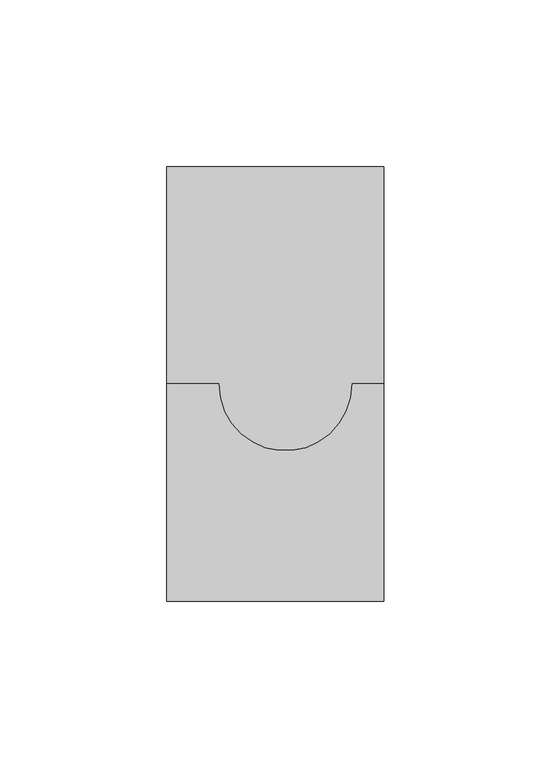
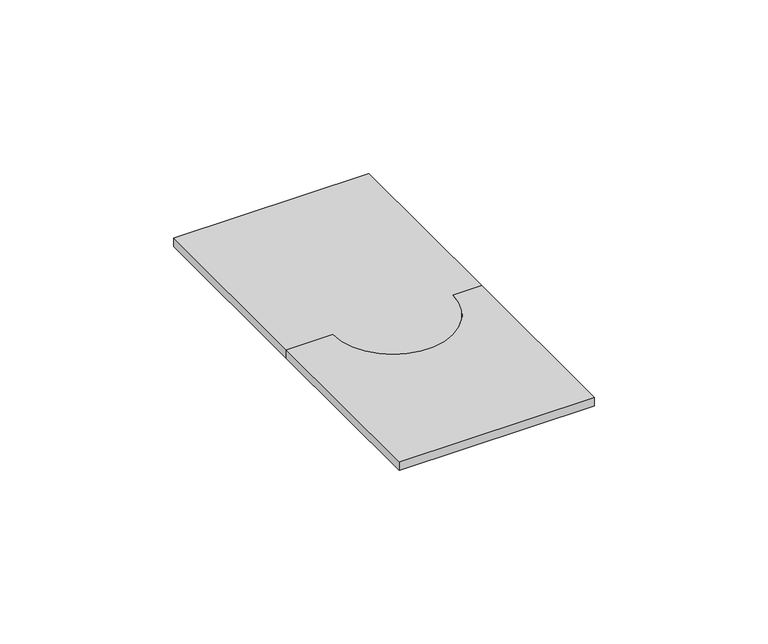
"""IFC4 building model written with IfcOpenShell, lengths in millimetres: proxy geometry, TSP Bonding & Earthing : TSP Bonding & Earthing."""

from ifc_helpers import new_model, si_unit, point, frame_2d, origin, origin_with_axes, place, context, project, spatial, polyline, circle_curve, trimmed, segment, composite_curve, outline, extrude, source, transform, mapped, element, save


def electrical_fixtures_1672ed60(model_context):
    return source(origin(), model_context, "Body", "SweptSolid", [
        extrude(outline(composite_curve([segment(polyline([(-9.5215648, 0.0), (0.0, 0.0), (0.0, -65.0), (-65.0, -65.0), (-65.0, 0.0), (-49.5215648, 0.0)]), True, "CONTINUOUS"), segment(trimmed(circle_curve(frame_2d((-29.5215648, 0.0)), 20.0), [point((-49.5215648, 0.0))], [point((-9.5215648, 0.0))], True, "CARTESIAN"), True, "CONTINUOUS")], self_intersect=False)), origin_with_axes(), (0.0, 0.0, 1.0), 3.0),
        extrude(outline(composite_curve([segment(trimmed(circle_curve(frame_2d((-29.5215648, 0.0)), 20.0), [point((-9.5215648, 0.0))], [point((-49.5215648, 0.0))], False, "CARTESIAN"), True, "CONTINUOUS"), segment(polyline([(-49.5215648, 0.0), (-65.0, 0.0), (-65.0, 65.0), (0.0, 65.0), (0.0, 0.0), (-9.5215648, 0.0)]), True, "CONTINUOUS")], self_intersect=False)), origin_with_axes(), (0.0, 0.0, 1.0), 3.0),
    ])


if __name__ == "__main__":
    model = new_model("IFC4")
    model_context = context("Model", 3, world=origin())
    ifc_project = project(units=[si_unit("LENGTHUNIT", "METRE", prefix="MILLI")], contexts=[model_context])
    site = spatial("IfcSite", under=ifc_project)
    building = spatial("IfcBuilding", under=site)
    placement = place(None, origin())
    electrical_fixtures_shape = electrical_fixtures_1672ed60(model_context)
    element("IfcBuildingElementProxy", 1, Name="TSP Bonding & Earthing : TSP Bonding & Earthing", ObjectType="TSP Bonding & Earthing : TSP Bonding & Earthing", at=placement, inside=building, context=model_context, shape_type="MappedRepresentation", body=[
        mapped(electrical_fixtures_shape, transform((0.0, 0.0, 0.0), x_axis=(1.0, 0.0, 0.0), y_axis=(0.0, 1.0, 0.0), z_axis=(0.0, 0.0, 1.0))),
    ])
    save(model, "model.ifc")

# Revit data of these elements
# Type "TSP Bonding & Earthing : TSP Bonding & Earthing"
#   Model = "TSP_ELECBNE"
#   Default Elevation = 0
# Element 1 (IfcBuildingElementProxy, "TSP Bonding & Earthing : TSP Bonding & Earthing")
#   Materials on its faces: "Plastic, Opaque Black", "Earth"
# Materials
#   "Plastic, Opaque Black": class "Plastic", colour RGB 0 0 0, transparency 0.7, Description = "Plastic, generic, opaque black", Cost = 0
#   "Earth": class "Generic", colour RGB 97 75 62, transparency 0, Description = "Soil", Cost = 0
